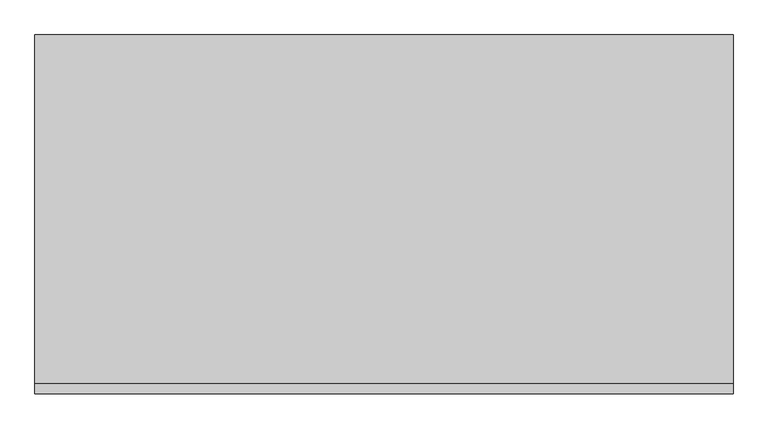
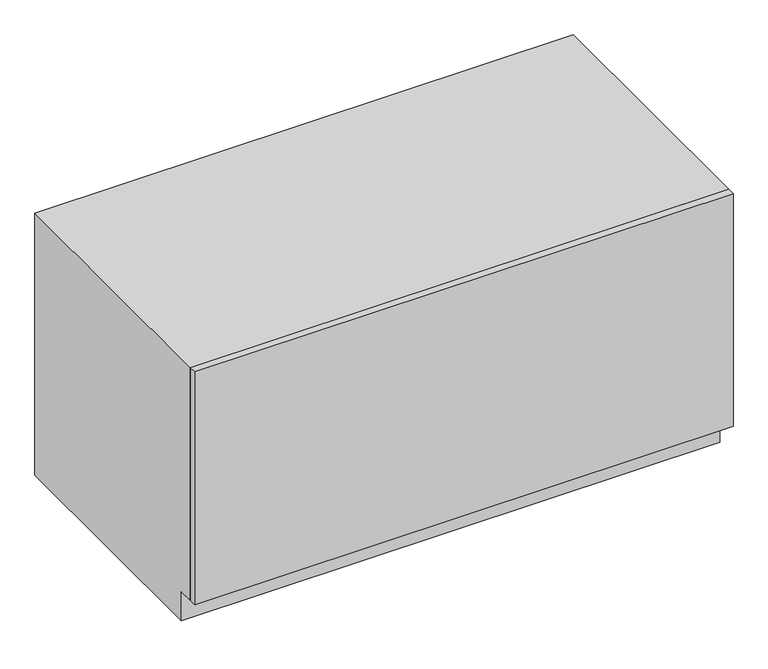
"""IFC4 building model written with IfcOpenShell, lengths in millimetres: furniture geometry, OD_CW_Base Cabinet : OD_CW_Base Cabinet."""

from ifc_helpers import new_model, si_unit, frame, origin, place, context, project, spatial, polyline, outline, extrude, source, transform, mapped, element, save


def furniture_76969ebe(model_context):
    return source(origin(), model_context, "Body", "SweptSolid", [
        extrude(outline(polyline([(18.7377049, -279.4), (1796.7377049, -279.4), (1796.7377049, -304.8), (18.7377049, -304.8), (18.7377049, -279.4)])), frame((0.0, 0.0, 101.6), z_axis=(0.0, 0.0, 1.0), x_axis=(1.0, 0.0, 0.0)), (0.0, 0.0, 1.0), 812.8),
        extrude(outline(polyline([(-279.4, 914.4), (609.6, 914.4), (609.6, 0.0), (-228.6, 0.0), (-228.6, 101.6), (-279.4, 101.6), (-279.4, 914.4)])), frame((18.7377049, 0.0, 0.0), z_axis=(1.0, 0.0, 0.0), x_axis=(0.0, 1.0, 0.0)), (0.0, 0.0, 1.0), 1778.0),
    ])


if __name__ == "__main__":
    model = new_model("IFC4")
    model_context = context("Model", 3, world=origin())
    ifc_project = project(units=[si_unit("LENGTHUNIT", "METRE", prefix="MILLI")], contexts=[model_context])
    site = spatial("IfcSite", under=ifc_project)
    building = spatial("IfcBuilding", under=site)
    placement = place(None, origin())
    furniture_shape = furniture_76969ebe(model_context)
    element("IfcFurniture", 1, ObjectType="OD_CW_Base Cabinet : OD_CW_Base Cabinet", at=placement, inside=building, context=model_context, shape_type="MappedRepresentation", body=[
        mapped(furniture_shape, transform((0.0, 0.0, 0.0), x_axis=(1.0, 0.0, 0.0), y_axis=(0.0, 1.0, 0.0), z_axis=(0.0, 0.0, 1.0))),
    ])
    save(model, "model.ifc")

# Revit data of these elements
# Type "OD_CW_Base Cabinet : OD_CW_Base Cabinet"
#   OD_CW_Width [instance default] = 2' - 10"
#   OD_CW_Length [instance default] = 8' - 0"
#   OD_CW_Height [instance default] = 2' - 3"
#   Depth = 2' - 0"
#   Height = 3' - 0"
#   Width = 4' - 0"
#   OD_CW_Material_Front Panel [instance default] = none
#   OD_CW_Material_Body [instance default] = none
# Element 1 (IfcFurniture, "OD_CW_Base Cabinet : OD_CW_Base Cabinet")
#   OD_CW_Width = 3' - 0"
#   OD_CW_Length = 5' - 10"
#   OD_CW_Height = 3' - 0"
#   OD_CW_Material_Body = PINSA PREP
#   Materials on its faces: "PINSA PREP", "CASEWORK"
# Materials
#   "PINSA PREP": class "Generic", colour RGB 187 187 187, transparency 0, Cost = 0
#   "CASEWORK": class "Generic", colour RGB 181 181 181, transparency 0, Cost = 0
